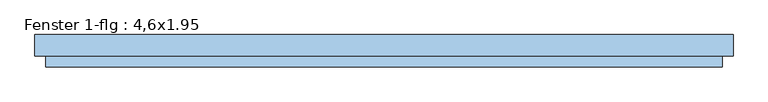
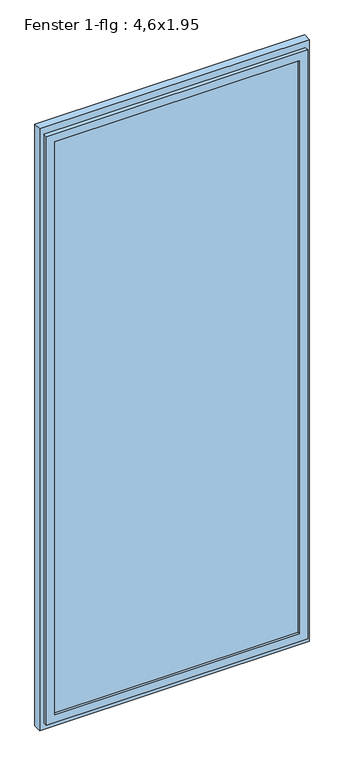
"""IFC4 building model written with IfcOpenShell, lengths in millimetres: window geometry, Fenster 1-flg : 4,6x1.95."""

import ifcopenshell
import ifcopenshell.guid

model = None  # the IFC model being written
_history = None  # IfcOwnerHistory: only IFC2X3 demands one
_inside = {}  # id of a spatial element -> (the spatial element, [elements in it])
_under = {}  # id of a project, library or spatial element -> (it, [spatial elements below it])
_declared = {}  # id of a project -> (the project, [libraries it declares])
_typed = {}  # id of a type object -> (the type object, [elements of that type])
_made_of = {}  # id of a material, layer set ... -> (it, [elements and type objects made of it])


def new_model(schema):
    """Start an empty IFC model of exactly this schema.

    Asked for "IFC4X3", IfcOpenShell would pick the latest addendum, in which some entities
    have other attributes; the version numbers below select the first issue.
    IFC2X3 requires an IfcOwnerHistory on every rooted entity: one is made here for all.
    """
    global model, _history
    if schema == "IFC4X3":
        model = ifcopenshell.file(schema_version=(4, 3, 0, 0))
    else:
        model = ifcopenshell.file(schema=schema)
    _inside.clear()
    _under.clear()
    _declared.clear()
    _typed.clear()
    _made_of.clear()
    _history = None
    if model.schema == "IFC2X3":
        org = make("IfcOrganization", Name="unknown")
        user = make(
            "IfcPersonAndOrganization",
            ThePerson=make("IfcPerson", FamilyName="unknown"),
            TheOrganization=org,
        )
        app = make(
            "IfcApplication",
            ApplicationDeveloper=org,
            Version="unknown",
            ApplicationFullName="unknown",
            ApplicationIdentifier="unknown",
        )
        _history = make(
            "IfcOwnerHistory",
            OwningUser=user,
            OwningApplication=app,
            ChangeAction="ADDED",
            CreationDate=0,
        )
    return model


def make(cls, **values):
    """One entity of the class cls with the attributes given. An attribute that is None is left unset."""
    return model.create_entity(
        cls, **{name: value for name, value in values.items() if value is not None}
    )


def rooted(cls, **values):
    """An entity with a GlobalId (a new one), such as an element, a storey or a relation."""
    return make(cls, GlobalId=ifcopenshell.guid.new(), OwnerHistory=_history, **values)


def si_unit(unit_type, name, prefix=None):
    """IfcSIUnit, for example si_unit("LENGTHUNIT", "METRE", prefix="MILLI")."""
    return make("IfcSIUnit", UnitType=unit_type, Prefix=prefix, Name=name)


def assignment(units):
    """IfcUnitAssignment: the units of a project."""
    return None if units is None else make("IfcUnitAssignment", Units=units)


def point(xyz):
    """IfcCartesianPoint."""
    return None if xyz is None else make("IfcCartesianPoint", Coordinates=xyz)


def direction(xyz):
    """IfcDirection."""
    return None if xyz is None else make("IfcDirection", DirectionRatios=xyz)


def frame(location, z_axis=None, x_axis=None):
    """IfcAxis2Placement3D, a coordinate frame: its origin and axes. An axis left out is left unset."""
    return make(
        "IfcAxis2Placement3D",
        Location=point(location),
        Axis=direction(z_axis),
        RefDirection=direction(x_axis),
    )


def origin():
    """The frame at (0, 0, 0) with its axes left unset."""
    return frame((0.0, 0.0, 0.0))


def place(relative_to, where):
    """IfcLocalPlacement: puts the frame where relative to a parent placement (None: the world)."""
    return make(
        "IfcLocalPlacement", PlacementRelTo=relative_to, RelativePlacement=where
    )


def context(
    kind, dimensions, precision=None, world=None, true_north=None, identifier=None
):
    """IfcGeometricRepresentationContext, for example the 3D "Model" context."""
    return make(
        "IfcGeometricRepresentationContext",
        ContextIdentifier=identifier,
        ContextType=kind,
        CoordinateSpaceDimension=dimensions,
        Precision=precision,
        WorldCoordinateSystem=world,
        TrueNorth=true_north,
    )


def project(units=None, contexts=None):
    """IfcProject with its units and contexts."""
    return rooted(
        "IfcProject",
        Name="project",
        RepresentationContexts=contexts,
        UnitsInContext=assignment(units),
    )


def spatial(cls, under=None, at=None, **own):
    """A site, building, storey or space (cls), placed at a placement, below another one or the project."""
    s = rooted(cls, ObjectPlacement=at, **own)
    if under is not None:
        _under.setdefault(under.id(), (under, []))[1].append(s)
    return s


def polyline(points):
    """IfcPolyline through the points."""
    return make("IfcPolyline", Points=[point(p) for p in points])


def outline(outer, holes=None, kind="AREA"):
    """IfcArbitraryClosedProfileDef: a profile drawn as a closed curve; with holes, ...WithVoids."""
    if holes is None:
        return make("IfcArbitraryClosedProfileDef", ProfileType=kind, OuterCurve=outer)
    return make(
        "IfcArbitraryProfileDefWithVoids",
        ProfileType=kind,
        OuterCurve=outer,
        InnerCurves=holes,
    )


def extrude(swept, where, along, depth):
    """IfcExtrudedAreaSolid: the profile swept, set in the frame where, extruded along a direction by depth."""
    return make(
        "IfcExtrudedAreaSolid",
        SweptArea=swept,
        Position=where,
        ExtrudedDirection=direction(along),
        Depth=depth,
    )


def faces_of(points, faces, orient=None, outer=None):
    """IfcFace entities. A face is a list of loops; a loop is a list of indices into points, from 0.

    orient and outer hold one flag for each loop. By default every Orientation is true, the
    first loop of a face is its IfcFaceOuterBound and the others are IfcFaceBound.
    """
    made = []
    for i, loops in enumerate(faces):
        bounds = []
        for j, loop in enumerate(loops):
            is_outer = j == 0 if outer is None else outer[i][j]
            bounds.append(
                make(
                    "IfcFaceOuterBound" if is_outer else "IfcFaceBound",
                    Bound=make("IfcPolyLoop", Polygon=[points[k] for k in loop]),
                    Orientation=True if orient is None else orient[i][j],
                )
            )
        made.append(make("IfcFace", Bounds=bounds))
    return made


def faceted_brep(points, faces, orient=None, outer=None, voids=None):
    """IfcFacetedBrep: a solid bounded by flat faces; with voids (closed shells), ...WithVoids."""
    shared = [point(p) for p in points]
    hull = make("IfcClosedShell", CfsFaces=faces_of(shared, faces, orient, outer))
    if voids is None:
        return make("IfcFacetedBrep", Outer=hull)
    return make(
        "IfcFacetedBrepWithVoids",
        Outer=hull,
        Voids=[
            make(cls, CfsFaces=faces_of(shared, fs, o, b)) for cls, fs, o, b in voids
        ],
    )


def shape(context_of_items, identifier, shape_type, items):
    """IfcShapeRepresentation: the items that make up one representation, for example the "Body"."""
    return make(
        "IfcShapeRepresentation",
        ContextOfItems=context_of_items,
        RepresentationIdentifier=identifier,
        RepresentationType=shape_type,
        Items=items,
    )


def source(mapping_origin, context_of_items, identifier, shape_type, items):
    """IfcRepresentationMap: a shape defined once, which mapped items show again and again."""
    return make(
        "IfcRepresentationMap",
        MappingOrigin=mapping_origin,
        MappedRepresentation=shape(context_of_items, identifier, shape_type, items),
    )


def transform(
    local_origin,
    x_axis=None,
    y_axis=None,
    z_axis=None,
    scale=None,
    scale2=None,
    scale3=None,
    uniform=True,
):
    """IfcCartesianTransformationOperator3D, or its non-uniform kind. x_axis, y_axis, z_axis: its Axis1, 2, 3."""
    if uniform:
        return make(
            "IfcCartesianTransformationOperator3D",
            Axis1=direction(x_axis),
            Axis2=direction(y_axis),
            LocalOrigin=point(local_origin),
            Scale=scale,
            Axis3=direction(z_axis),
        )
    return make(
        "IfcCartesianTransformationOperator3DnonUniform",
        Axis1=direction(x_axis),
        Axis2=direction(y_axis),
        LocalOrigin=point(local_origin),
        Scale=scale,
        Axis3=direction(z_axis),
        Scale2=scale2,
        Scale3=scale3,
    )


def mapped(mapping_source, mapping_target):
    """IfcMappedItem: shows the shape of a source again, moved by a transform."""
    return make(
        "IfcMappedItem", MappingSource=mapping_source, MappingTarget=mapping_target
    )


def made_of(thing, what):
    """Note that an element or type object is made of a material, layer set ...; save() writes the relation."""
    if what is not None:
        _made_of.setdefault(what.id(), (what, []))[1].append(thing)
    return thing


def element(
    cls,
    number,
    at=None,
    inside=None,
    cuts=None,
    type_object=None,
    material=None,
    context=None,
    identifier="Body",
    shape_type=None,
    held_by="IfcProductDefinitionShape",
    body=None,
    shapes=None,
    **own,
):
    """One element of the class cls, such as IfcWall. Its Tag is "e" and its number.

    at: its placement. inside: the storey or other place that contains it. cuts: it is an
    opening in that element (IfcRelVoidsElement). A single representation is given by context,
    identifier, shape_type and body (its items); several are given by shapes. held_by: the class
    of the entity that holds the representations. save() writes the other relations.
    """
    e = rooted(cls, Tag="e%d" % number, ObjectPlacement=at, **own)
    if body is not None:
        shapes = [shape(context, identifier, shape_type, body)]
    if shapes is not None:
        e.Representation = make(held_by, Representations=shapes)
    if inside is not None:
        _inside.setdefault(inside.id(), (inside, []))[1].append(e)
    if cuts is not None:
        rooted(
            "IfcRelVoidsElement", RelatingBuildingElement=cuts, RelatedOpeningElement=e
        )
    if type_object is not None:
        _typed.setdefault(type_object.id(), (type_object, []))[1].append(e)
    return made_of(e, material)


def aggregate(whole, parts):
    """IfcRelAggregates: a whole, such as a stair, and the parts it consists of."""
    return rooted("IfcRelAggregates", RelatingObject=whole, RelatedObjects=parts)


def save(model, path):
    """Write the relations noted so far, then the file.

    IfcRelAggregates (storeys below a building ...), IfcRelContainedInSpatialStructure (elements
    in a storey), IfcRelDefinesByType, IfcRelAssociatesMaterial and IfcRelDeclares: one each for
    every whole, place, type object, material and project.
    """
    for whole, parts in _under.values():
        aggregate(whole, parts)
    for where, things in _inside.values():
        rooted(
            "IfcRelContainedInSpatialStructure",
            RelatedElements=things,
            RelatingStructure=where,
        )
    for kind, things in _typed.values():
        rooted("IfcRelDefinesByType", RelatedObjects=things, RelatingType=kind)
    for what, things in _made_of.values():
        rooted("IfcRelAssociatesMaterial", RelatedObjects=things, RelatingMaterial=what)
    for by, libraries in _declared.values():
        rooted("IfcRelDeclares", RelatingContext=by, RelatedDefinitions=libraries)
    model.write(path)


def fenster_1_flg_4_6x1_95_63455175(model_context):
    return source(origin(), model_context, "Body", "SolidModel", [
        extrude(outline(polyline([(5600.0, 975.0), (5600.0, -975.0), (1000.0, -975.0), (1000.0, 975.0), (5600.0, 975.0)]), holes=[polyline([(5520.0, 915.0), (1080.0, 915.0), (1080.0, -915.0), (5520.0, -915.0), (5520.0, 915.0)])]), frame((0.0, 20.0, 0.0), z_axis=(0.0, 1.0, 0.0), x_axis=(0.0, 0.0, 1.0)), (0.0, 0.0, 1.0), 60.0),
        faceted_brep([(945.0, 20.0, 5550.0), (945.0, -10.0, 5550.0), (945.0, -10.0, 1050.0), (945.0, 20.0, 1050.0), (-945.0, -10.0, 5550.0), (-945.0, -10.0, 1050.0), (885.0, -10.0, 1110.0), (-885.0, -10.0, 1110.0), (-885.0, -10.0, 5490.0), (885.0, -10.0, 5490.0), (-945.0, 20.0, 1050.0), (-945.0, 20.0, 5550.0), (915.0, 20.0, 5520.0), (-915.0, 20.0, 5520.0), (-915.0, 20.0, 1080.0), (915.0, 20.0, 1080.0), (915.0, 50.0, 5520.0), (915.0, 50.0, 1080.0), (-915.0, 50.0, 1080.0), (-915.0, 50.0, 5520.0), (885.0, 50.0, 5490.0), (-885.0, 50.0, 5490.0), (-885.0, 50.0, 1110.0), (885.0, 50.0, 1110.0)], [[[0, 1, 2, 3]], [[1, 4, 5, 2], [6, 7, 8, 9]], [[3, 2, 5, 10]], [[3, 10, 11, 0], [12, 13, 14, 15]], [[16, 12, 15, 17]], [[17, 15, 14, 18]], [[17, 18, 19, 16], [20, 21, 22, 23]], [[9, 20, 23, 6]], [[6, 23, 22, 7]], [[10, 5, 4, 11]], [[18, 14, 13, 19]], [[7, 22, 21, 8]], [[11, 4, 1, 0]], [[19, 13, 12, 16]], [[8, 21, 20, 9]]]),
        extrude(outline(polyline([(885.0, 5.0), (-885.0, 5.0), (-885.0, 35.0), (885.0, 35.0), (885.0, 5.0)])), frame((0.0, 0.0, 1110.0), z_axis=(0.0, 0.0, 1.0), x_axis=(1.0, 0.0, 0.0)), (0.0, 0.0, 1.0), 4380.0),
    ])


if __name__ == "__main__":
    model = new_model("IFC4")
    model_context = context("Model", 3, world=origin())
    ifc_project = project(units=[si_unit("LENGTHUNIT", "METRE", prefix="MILLI")], contexts=[model_context])
    site = spatial("IfcSite", under=ifc_project)
    building = spatial("IfcBuilding", under=site)
    placement = place(None, origin())
    fenster_1_flg_4_6x1_95_shape = fenster_1_flg_4_6x1_95_63455175(model_context)
    element("IfcWindow", 1, ObjectType="Fenster 1-flg : 4,6x1.95", at=placement, inside=building, context=model_context, shape_type="MappedRepresentation", body=[
        mapped(fenster_1_flg_4_6x1_95_shape, transform((0.0, 0.0, 0.0), x_axis=(1.0, 0.0, 0.0), y_axis=(0.0, 1.0, 0.0), z_axis=(0.0, 0.0, 1.0))),
    ])
    save(model, "model.ifc")

# Revit data of these elements
# Type "Fenster 1-flg : 4,6x1.95"
#   Type Mark = "61"
#   Operation = "SinglePanel"
#   Keynote = "16.05.01"
#   Visual Light Transmittance = 0.9
#   Solar Heat Gain Coefficient = 0.86
#   Rough Width = 1.950 m
#   Rough Height = 4.600 m
#   Heat Transfer Coefficient (U) = 5.5617 W/(m²·K)
#   Rahmentiefe = 0.060 m
#   Rahmenhöhe - unten = 0.080 m
#   Rahmenhöhe - oben = 0.080 m
#   Rahmenbreite = 0.060 m
#   Height = 4.600 m
#   Tiefe Flügel = 0.060 m
#   Flügelbreite = 0.060 m
#   Einbautiefe (von außen) [instance default] = 0.100 m
#   Width = 1.950 m
#   Klappflügel [instance default] = no
#   Kippflügel [instance default] = yes
#   Öffnungsrichtung in Draufsicht anzeigen [instance default] = no
#   Drehflügel 1 [instance default] = yes
#   Rahmen 1 [instance default] = none
#   Glas [instance default] = none
#   Flügel [instance default] = none
#   Fensterbank Innenseite [instance default] = none
#   Fensterbank Außenseite [instance default] = none
#   Construction Type Id = ""
#   Wall Closure = (empty or 0)
#   Analytic Construction = (empty or 0)
# Element 1 (IfcWindow, "Fenster 1-flg : 4,6x1.95")
#   Einbautiefe (von außen) = 0.230 m
#   Materials on its faces: "Kunststoff - Weiß", "Glas"
# Materials
#   "Kunststoff - Weiß": class "Kunststoff", colour RGB 249 249 249, transparency 0, Cost = 0
#   "Glas": class "Glas", colour RGB 0 0 255, transparency 0.75, Comments = "Render-Darstellung nicht aktualisiert ", Cost = 0
